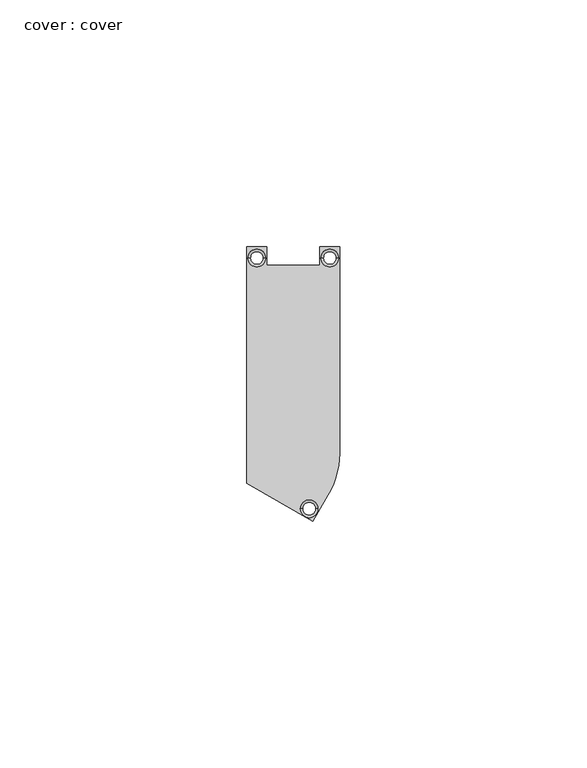
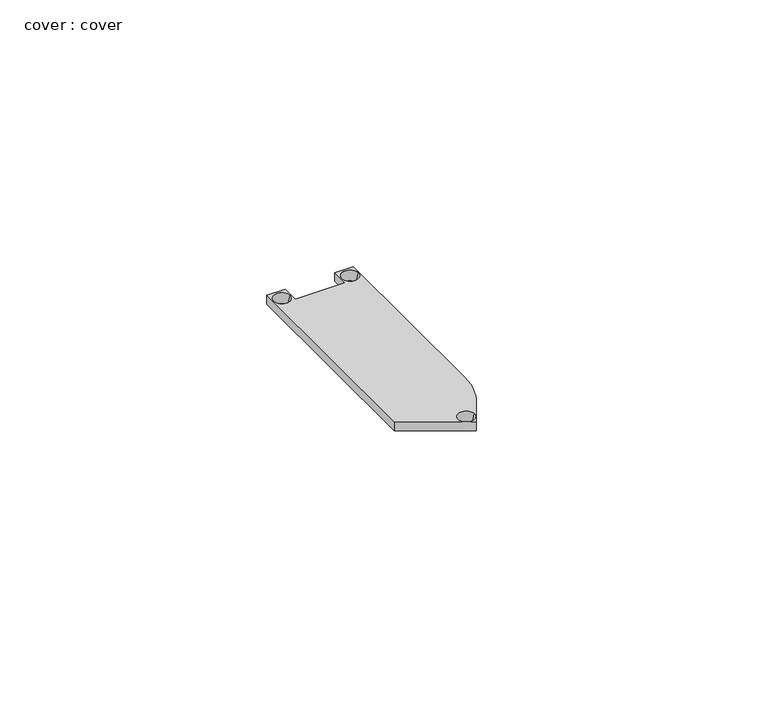
"""IFC4 building model written with IfcOpenShell, lengths in millimetres: proxy geometry, cover : cover."""

from ifc_helpers import new_model, si_unit, frame, origin, place, context, project, spatial, polyline, circle_curve, source, transform, mapped, element, save
from ifc_brep_helpers import plane_surface, revolved_surface, advanced_brep


def cover_cover_cea35c0b(model_context):
    return source(origin(), model_context, "Body", "AdvancedBrep", [
        advanced_brep(
        [(4663.3311724, 3578.6670305, 2.0), (4663.3311724, 3530.8564939, 2.0), (4676.6686902, 3523.1530364, 2.0), (4680.3669524, 3529.5586705, 2.0), (4680.8851124, 3530.7118305, 2.0), (4681.3143724, 3531.9030905, 2.0), (4681.6547324, 3533.1222905, 2.0), (4681.9011124, 3534.3618105, 2.0), (4682.0560524, 3535.6191105, 2.0), (4682.1119324, 3536.8840305, 2.0), (4682.1119324, 3578.6670305, 2.0), (4678.1114324, 3578.6670305, 2.0), (4678.1114324, 3574.9179905, 2.0), (4667.3316724, 3574.9179905, 2.0), (4667.3316724, 3578.6670305, 2.0), (4667.1314224, 3576.4165905, 2.0), (4663.5314224, 3576.4165905, 2.0), (4681.9129524, 3576.4165905, 2.0), (4678.3129524, 3576.4165905, 2.0), (4677.7131366, 3525.6369105, 2.0), (4674.1587083, 3525.6369105, 2.0), (4663.3311724, 3578.6670305, 0.0), (4667.3316724, 3578.6670305, 0.0), (4667.3316724, 3574.9179905, 0.0), (4678.1114324, 3574.9179905, 0.0), (4678.1114324, 3578.6670305, 0.0), (4682.1119324, 3578.6670305, 0.0), (4682.1119324, 3536.8840305, 0.0), (4682.0560524, 3535.6191105, 0.0), (4681.9011124, 3534.3618105, 0.0), (4681.6547324, 3533.1222905, 0.0), (4681.3143724, 3531.9030905, 0.0), (4680.8851124, 3530.7118305, 0.0), (4680.3669524, 3529.5586705, 0.0), (4676.6686902, 3523.1530364, 0.0), (4663.3311724, 3530.8564939, 0.0), (4664.0314224, 3576.4165905, 0.0), (4666.6314224, 3576.4165905, 0.0), (4678.8129524, 3576.4165905, 0.0), (4681.4129524, 3576.4165905, 0.0), (4674.6206691, 3525.6369105, 0.0), (4677.2511758, 3525.6369105, 0.0)],
        [
            (0, 1),
            (1, 2),
            (2, 3),
            (3, 4),
            (4, 5),
            (5, 6),
            (6, 7),
            (7, 8),
            (8, 9),
            (9, 10),
            (10, 11),
            (11, 12),
            (12, 13),
            (13, 14),
            (14, 0),
            (15, 16, circle_curve(frame((4665.3314224, 3576.4165905, 2.0), z_axis=(0.0, 0.0, -1.0), x_axis=(-1.0, 0.0, 0.0)), 1.8)),
            (16, 15, circle_curve(frame((4665.3314224, 3576.4165905, 2.0), z_axis=(0.0, 0.0, -1.0), x_axis=(1.0, 0.0, 0.0)), 1.8)),
            (17, 18, circle_curve(frame((4680.1129524, 3576.4165905, 2.0), z_axis=(0.0, 0.0, -1.0), x_axis=(-1.0, 0.0, 0.0)), 1.8)),
            (18, 17, circle_curve(frame((4680.1129524, 3576.4165905, 2.0), z_axis=(0.0, 0.0, -1.0), x_axis=(1.0, 0.0, 0.0)), 1.8)),
            (19, 20, circle_curve(frame((4675.9359224, 3525.6369105, 2.0), z_axis=(0.0, 0.0, -1.0), x_axis=(-1.0, 0.0, 0.0)), 1.7772142)),
            (20, 19, circle_curve(frame((4675.9359224, 3525.6369105, 2.0), z_axis=(0.0, 0.0, -1.0), x_axis=(1.0, 0.0, 0.0)), 1.7772142)),
            (21, 22),
            (22, 23),
            (23, 24),
            (24, 25),
            (25, 26),
            (26, 27),
            (27, 28),
            (28, 29),
            (29, 30),
            (30, 31),
            (31, 32),
            (32, 33),
            (33, 34),
            (34, 35),
            (35, 21),
            (36, 37, circle_curve(frame((4665.3314224, 3576.4165905, 0.0), z_axis=(0.0, 0.0, 1.0), x_axis=(-1.0, 0.0, 0.0)), 1.3)),
            (37, 36, circle_curve(frame((4665.3314224, 3576.4165905, 0.0), z_axis=(0.0, 0.0, 1.0), x_axis=(1.0, 0.0, 0.0)), 1.3)),
            (38, 39, circle_curve(frame((4680.1129524, 3576.4165905, 0.0), z_axis=(0.0, 0.0, 1.0), x_axis=(-1.0, 0.0, 0.0)), 1.3)),
            (39, 38, circle_curve(frame((4680.1129524, 3576.4165905, 0.0), z_axis=(0.0, 0.0, 1.0), x_axis=(1.0, 0.0, 0.0)), 1.3)),
            (40, 41, circle_curve(frame((4675.9359224, 3525.6369105, 0.0), z_axis=(0.0, 0.0, 1.0), x_axis=(-1.0, 0.0, 0.0)), 1.3152534)),
            (41, 40, circle_curve(frame((4675.9359224, 3525.6369105, 0.0), z_axis=(0.0, 0.0, 1.0), x_axis=(1.0, 0.0, 0.0)), 1.3152534)),
            (0, 21),
            (35, 1),
            (34, 2),
            (33, 3),
            (9, 27),
            (26, 10),
            (32, 4),
            (31, 5),
            (30, 6),
            (29, 7),
            (28, 8),
            (25, 11),
            (36, 16),
            (15, 37),
            (38, 18),
            (17, 39),
            (40, 20),
            (19, 41),
            (24, 12),
            (23, 13),
            (22, 14),
        ],
        [
            plane_surface(frame((4663.3311724, 3531.8548305, 2.0), z_axis=(0.0, 0.0, 1.0), x_axis=(0.0, -1.0, 0.0))),
            plane_surface(frame((4663.3311724, 3531.8548305, 0.0), z_axis=(0.0, 0.0, -1.0), x_axis=(0.0, 1.0, 0.0))),
            plane_surface(frame((4663.3311724, 3578.6670305, 2.0), z_axis=(-1.0, 0.0, 0.0), x_axis=(0.0, 0.0, -1.0))),
            plane_surface(frame((4663.3311724, 3530.8564939, 2.0), z_axis=(-0.5001479267947955, -0.8659399813629511, 0.0), x_axis=(0.0, 0.0, -1.0))),
            plane_surface(frame((4676.6686902, 3523.1530364, 2.0), z_axis=(0.8660272939548818, -0.49999672611446655, 0.0), x_axis=(0.0, 0.0, -1.0))),
            plane_surface(frame((4682.1119324, 3536.8840305, 2.0), z_axis=(1.0, 0.0, 0.0), x_axis=(0.0, 0.0, -1.0))),
            plane_surface(frame((4680.3669524, 3529.5586705, 2.0), z_axis=(0.91214692510674, -0.40986337603928397, 0.0), x_axis=(0.0, 0.0, -1.0))),
            plane_surface(frame((4680.8851124, 3530.7118305, 2.0), z_axis=(0.9407850831608502, -0.3390035800725891, 0.0), x_axis=(0.0, 0.0, -1.0))),
            plane_surface(frame((4681.3143724, 3531.9030905, 2.0), z_axis=(0.9631721335643817, -0.26888555395379093, 0.0), x_axis=(0.0, 0.0, -1.0))),
            plane_surface(frame((4681.6547324, 3533.1222905, 2.0), z_axis=(0.9808118970912181, -0.19495646315094542, 0.0), x_axis=(0.0, 0.0, -1.0))),
            plane_surface(frame((4681.9011124, 3534.3618105, 2.0), z_axis=(0.9924922999614717, -0.12230713191465294, 0.0), x_axis=(0.0, 0.0, -1.0))),
            plane_surface(frame((4682.0560524, 3535.6191105, 2.0), z_axis=(0.9990256352193916, -0.04413366260000536, 0.0), x_axis=(0.0, 0.0, -1.0))),
            plane_surface(frame((4682.1119324, 3578.6670305, 2.0), z_axis=(0.0, 1.0, 0.0), x_axis=(0.0, 0.0, -1.0))),
            revolved_surface(polyline([(4663.5314224, 3576.4165905, 2.0), (4664.0314224, 3576.4165905, 0.0)]), (4665.3314224, 3576.4165905, -5.2), (0.0, 0.0, 1.0)),
            revolved_surface(polyline([(4678.3129524, 3576.4165905, 2.0), (4678.8129524, 3576.4165905, 0.0)]), (4680.1129524, 3576.4165905, -5.2), (0.0, 0.0, 1.0)),
            revolved_surface(polyline([(4674.1587083, 3525.6369105, 2.0), (4674.620669086516, 3525.6369105, 0.0)]), (4675.9359224, 3525.6369105, -5.6942206), (0.0, 0.0, 1.0)),
            plane_surface(frame((4678.1114324, 3578.6670305, 2.0), z_axis=(-1.0, 0.0, 0.0), x_axis=(0.0, 0.0, -1.0))),
            plane_surface(frame((4678.1114324, 3574.9179905, 2.0), z_axis=(0.0, 1.0, 0.0), x_axis=(0.0, 0.0, -1.0))),
            plane_surface(frame((4667.3316724, 3574.9179905, 2.0), z_axis=(1.0, 0.0, 0.0), x_axis=(0.0, 0.0, -1.0))),
            plane_surface(frame((4667.3316724, 3578.6670305, 2.0), z_axis=(0.0, 1.0, 0.0), x_axis=(0.0, 0.0, -1.0))),
        ],
        [
            (0, [[1, 2, 3, 4, 5, 6, 7, 8, 9, 10, 11, 12, 13, 14, 15], [16, 17], [18, 19], [20, 21]]),
            (1, [[22, 23, 24, 25, 26, 27, 28, 29, 30, 31, 32, 33, 34, 35, 36], [37, 38], [39, 40], [41, 42]]),
            (2, [[-1, 43, -36, 44]]),
            (3, [[-2, -44, -35, 45]]),
            (4, [[-3, -45, -34, 46]]),
            (5, [[-10, 47, -27, 48]]),
            (6, [[-4, -46, -33, 49]]),
            (7, [[-5, -49, -32, 50]]),
            (8, [[-6, -50, -31, 51]]),
            (9, [[-7, -51, -30, 52]]),
            (10, [[-8, -52, -29, 53]]),
            (11, [[-9, -53, -28, -47]]),
            (12, [[-11, -48, -26, 54]]),
            (13, [[55, -16, 56, -37]]),
            (13, [[-55, -38, -56, -17]]),
            (14, [[57, -18, 58, -39]]),
            (14, [[-57, -40, -58, -19]]),
            (15, [[59, -20, 60, -41]]),
            (15, [[-59, -42, -60, -21]]),
            (16, [[-12, -54, -25, 61]]),
            (17, [[-13, -61, -24, 62]]),
            (18, [[-14, -62, -23, 63]]),
            (19, [[-15, -63, -22, -43]]),
        ],
    ),
    ])


if __name__ == "__main__":
    model = new_model("IFC4")
    model_context = context("Model", 3, world=origin())
    ifc_project = project(units=[si_unit("LENGTHUNIT", "METRE", prefix="MILLI")], contexts=[model_context])
    site = spatial("IfcSite", under=ifc_project)
    building = spatial("IfcBuilding", under=site)
    placement = place(None, origin())
    cover_cover_shape = cover_cover_cea35c0b(model_context)
    element("IfcBuildingElementProxy", 1, Name="cover : cover", ObjectType="cover : cover", at=placement, inside=building, context=model_context, shape_type="MappedRepresentation", body=[
        mapped(cover_cover_shape, transform((0.0, 0.0, 0.0), x_axis=(1.0, 0.0, 0.0), y_axis=(0.0, 1.0, 0.0), z_axis=(0.0, 0.0, 1.0))),
    ])
    save(model, "model.ifc")
